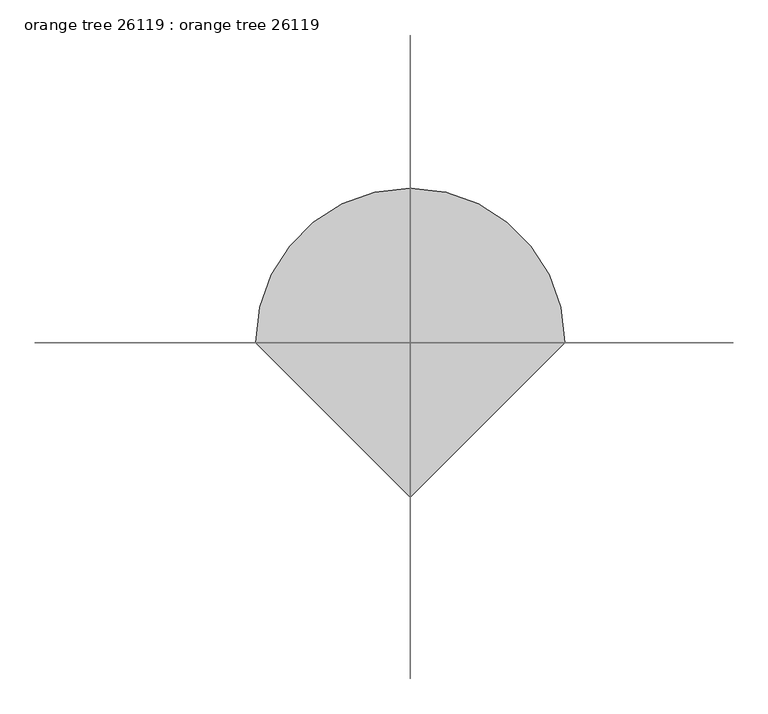
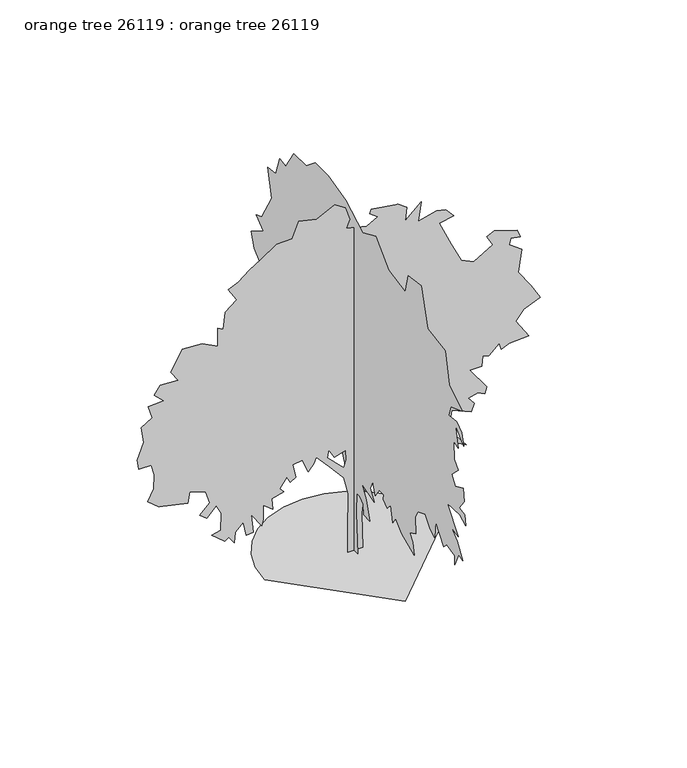
"""IFC4 building model written with IfcOpenShell, lengths in millimetres: proxy geometry, orange tree 26119 : orange tree 26119."""

import ifcopenshell
import ifcopenshell.guid

model = None  # the IFC model being written
_history = None  # IfcOwnerHistory: only IFC2X3 demands one
_inside = {}  # id of a spatial element -> (the spatial element, [elements in it])
_under = {}  # id of a project, library or spatial element -> (it, [spatial elements below it])
_declared = {}  # id of a project -> (the project, [libraries it declares])
_typed = {}  # id of a type object -> (the type object, [elements of that type])
_made_of = {}  # id of a material, layer set ... -> (it, [elements and type objects made of it])


def new_model(schema):
    """Start an empty IFC model of exactly this schema.

    Asked for "IFC4X3", IfcOpenShell would pick the latest addendum, in which some entities
    have other attributes; the version numbers below select the first issue.
    IFC2X3 requires an IfcOwnerHistory on every rooted entity: one is made here for all.
    """
    global model, _history
    if schema == "IFC4X3":
        model = ifcopenshell.file(schema_version=(4, 3, 0, 0))
    else:
        model = ifcopenshell.file(schema=schema)
    _inside.clear()
    _under.clear()
    _declared.clear()
    _typed.clear()
    _made_of.clear()
    _history = None
    if model.schema == "IFC2X3":
        org = make("IfcOrganization", Name="unknown")
        user = make(
            "IfcPersonAndOrganization",
            ThePerson=make("IfcPerson", FamilyName="unknown"),
            TheOrganization=org,
        )
        app = make(
            "IfcApplication",
            ApplicationDeveloper=org,
            Version="unknown",
            ApplicationFullName="unknown",
            ApplicationIdentifier="unknown",
        )
        _history = make(
            "IfcOwnerHistory",
            OwningUser=user,
            OwningApplication=app,
            ChangeAction="ADDED",
            CreationDate=0,
        )
    return model


def make(cls, **values):
    """One entity of the class cls with the attributes given. An attribute that is None is left unset."""
    return model.create_entity(
        cls, **{name: value for name, value in values.items() if value is not None}
    )


def rooted(cls, **values):
    """An entity with a GlobalId (a new one), such as an element, a storey or a relation."""
    return make(cls, GlobalId=ifcopenshell.guid.new(), OwnerHistory=_history, **values)


def si_unit(unit_type, name, prefix=None):
    """IfcSIUnit, for example si_unit("LENGTHUNIT", "METRE", prefix="MILLI")."""
    return make("IfcSIUnit", UnitType=unit_type, Prefix=prefix, Name=name)


def assignment(units):
    """IfcUnitAssignment: the units of a project."""
    return None if units is None else make("IfcUnitAssignment", Units=units)


def point(xyz):
    """IfcCartesianPoint."""
    return None if xyz is None else make("IfcCartesianPoint", Coordinates=xyz)


def direction(xyz):
    """IfcDirection."""
    return None if xyz is None else make("IfcDirection", DirectionRatios=xyz)


def frame(location, z_axis=None, x_axis=None):
    """IfcAxis2Placement3D, a coordinate frame: its origin and axes. An axis left out is left unset."""
    return make(
        "IfcAxis2Placement3D",
        Location=point(location),
        Axis=direction(z_axis),
        RefDirection=direction(x_axis),
    )


def origin():
    """The frame at (0, 0, 0) with its axes left unset."""
    return frame((0.0, 0.0, 0.0))


def place(relative_to, where):
    """IfcLocalPlacement: puts the frame where relative to a parent placement (None: the world)."""
    return make(
        "IfcLocalPlacement", PlacementRelTo=relative_to, RelativePlacement=where
    )


def context(
    kind, dimensions, precision=None, world=None, true_north=None, identifier=None
):
    """IfcGeometricRepresentationContext, for example the 3D "Model" context."""
    return make(
        "IfcGeometricRepresentationContext",
        ContextIdentifier=identifier,
        ContextType=kind,
        CoordinateSpaceDimension=dimensions,
        Precision=precision,
        WorldCoordinateSystem=world,
        TrueNorth=true_north,
    )


def project(units=None, contexts=None):
    """IfcProject with its units and contexts."""
    return rooted(
        "IfcProject",
        Name="project",
        RepresentationContexts=contexts,
        UnitsInContext=assignment(units),
    )


def spatial(cls, under=None, at=None, **own):
    """A site, building, storey or space (cls), placed at a placement, below another one or the project."""
    s = rooted(cls, ObjectPlacement=at, **own)
    if under is not None:
        _under.setdefault(under.id(), (under, []))[1].append(s)
    return s


def point_list(points):
    """IfcCartesianPointList2D or 3D."""
    cls = (
        "IfcCartesianPointList2D" if len(points[0]) == 2 else "IfcCartesianPointList3D"
    )
    return make(cls, CoordList=points)


def triangles(points, corners, closed=None, point_numbers=None):
    """IfcTriangulatedFaceSet: each triangle names its three corners, points numbered from 1."""
    return make(
        "IfcTriangulatedFaceSet",
        Coordinates=point_list(points),
        Closed=closed,
        CoordIndex=corners,
        PnIndex=point_numbers,
    )


def shape(context_of_items, identifier, shape_type, items):
    """IfcShapeRepresentation: the items that make up one representation, for example the "Body"."""
    return make(
        "IfcShapeRepresentation",
        ContextOfItems=context_of_items,
        RepresentationIdentifier=identifier,
        RepresentationType=shape_type,
        Items=items,
    )


def source(mapping_origin, context_of_items, identifier, shape_type, items):
    """IfcRepresentationMap: a shape defined once, which mapped items show again and again."""
    return make(
        "IfcRepresentationMap",
        MappingOrigin=mapping_origin,
        MappedRepresentation=shape(context_of_items, identifier, shape_type, items),
    )


def transform(
    local_origin,
    x_axis=None,
    y_axis=None,
    z_axis=None,
    scale=None,
    scale2=None,
    scale3=None,
    uniform=True,
):
    """IfcCartesianTransformationOperator3D, or its non-uniform kind. x_axis, y_axis, z_axis: its Axis1, 2, 3."""
    if uniform:
        return make(
            "IfcCartesianTransformationOperator3D",
            Axis1=direction(x_axis),
            Axis2=direction(y_axis),
            LocalOrigin=point(local_origin),
            Scale=scale,
            Axis3=direction(z_axis),
        )
    return make(
        "IfcCartesianTransformationOperator3DnonUniform",
        Axis1=direction(x_axis),
        Axis2=direction(y_axis),
        LocalOrigin=point(local_origin),
        Scale=scale,
        Axis3=direction(z_axis),
        Scale2=scale2,
        Scale3=scale3,
    )


def mapped(mapping_source, mapping_target):
    """IfcMappedItem: shows the shape of a source again, moved by a transform."""
    return make(
        "IfcMappedItem", MappingSource=mapping_source, MappingTarget=mapping_target
    )


def made_of(thing, what):
    """Note that an element or type object is made of a material, layer set ...; save() writes the relation."""
    if what is not None:
        _made_of.setdefault(what.id(), (what, []))[1].append(thing)
    return thing


def element(
    cls,
    number,
    at=None,
    inside=None,
    cuts=None,
    type_object=None,
    material=None,
    context=None,
    identifier="Body",
    shape_type=None,
    held_by="IfcProductDefinitionShape",
    body=None,
    shapes=None,
    **own,
):
    """One element of the class cls, such as IfcWall. Its Tag is "e" and its number.

    at: its placement. inside: the storey or other place that contains it. cuts: it is an
    opening in that element (IfcRelVoidsElement). A single representation is given by context,
    identifier, shape_type and body (its items); several are given by shapes. held_by: the class
    of the entity that holds the representations. save() writes the other relations.
    """
    e = rooted(cls, Tag="e%d" % number, ObjectPlacement=at, **own)
    if body is not None:
        shapes = [shape(context, identifier, shape_type, body)]
    if shapes is not None:
        e.Representation = make(held_by, Representations=shapes)
    if inside is not None:
        _inside.setdefault(inside.id(), (inside, []))[1].append(e)
    if cuts is not None:
        rooted(
            "IfcRelVoidsElement", RelatingBuildingElement=cuts, RelatedOpeningElement=e
        )
    if type_object is not None:
        _typed.setdefault(type_object.id(), (type_object, []))[1].append(e)
    return made_of(e, material)


def aggregate(whole, parts):
    """IfcRelAggregates: a whole, such as a stair, and the parts it consists of."""
    return rooted("IfcRelAggregates", RelatingObject=whole, RelatedObjects=parts)


def save(model, path):
    """Write the relations noted so far, then the file.

    IfcRelAggregates (storeys below a building ...), IfcRelContainedInSpatialStructure (elements
    in a storey), IfcRelDefinesByType, IfcRelAssociatesMaterial and IfcRelDeclares: one each for
    every whole, place, type object, material and project.
    """
    for whole, parts in _under.values():
        aggregate(whole, parts)
    for where, things in _inside.values():
        rooted(
            "IfcRelContainedInSpatialStructure",
            RelatedElements=things,
            RelatingStructure=where,
        )
    for kind, things in _typed.values():
        rooted("IfcRelDefinesByType", RelatedObjects=things, RelatingType=kind)
    for what, things in _made_of.values():
        rooted("IfcRelAssociatesMaterial", RelatedObjects=things, RelatingMaterial=what)
    for by, libraries in _declared.values():
        rooted("IfcRelDeclares", RelatingContext=by, RelatedDefinitions=libraries)
    model.write(path)


def orange_tree_26119_orange_tree_26119_f1cce5cf(model_context):
    return source(origin(), model_context, "Body", "Tessellation", [
        triangles([(-803.9534712, 0.0, 6.05e-05), (-782.6987366, 184.2127929, 6.05e-05), (-722.1679836, 353.3826814, 6.05e-05), (-627.2075008, 502.663613, 6.05e-05), (-502.663613, 627.2075008, 6.05e-05), (-353.3826814, 722.1679836, 6.05e-05), (-184.2125386, 782.6987366, 6.05e-05), (3.51e-05, 803.9534712, 6.05e-05), (184.2127929, 782.6987366, 6.05e-05), (353.3826814, 722.1679836, 6.05e-05), (502.663613, 627.2075008, 6.05e-05), (627.2075008, 502.663613, 6.05e-05), (722.1679836, 353.3826814, 6.05e-05), (782.6987366, 184.2125386, 6.05e-05), (803.9534712, -7.03e-05, 6.05e-05), (-0.0001054, -803.9534712, 6.05e-05), (-4.73e-05, 77.0963933, 4.81e-05), (-2.95e-05, 72.7562921, 588.9525321), (-2.7e-05, 181.2628458, 836.3460434), (-3.2e-05, 320.1518609, 875.4087753), (-3.63e-05, 346.1919502, 771.2433311), (-3.87e-05, 472.0617019, 879.7495714), (-4.71e-05, 532.8235817, 688.7770712), (-4.92e-05, 632.6507006, 766.9024624), (-5.78e-05, 693.4151602, 571.5916368), (-5.81e-05, 775.878804, 684.4387459), (-6.3e-05, 832.3023949, 606.3134274), (-6.59e-05, 979.8713671, 727.8398031), (-5.62e-05, 875.7059229, 897.110503), (-4.32e-05, 610.9489002, 936.1731623), (-5.12e-05, 849.6633265, 1027.3185436), (-5.75e-05, 1031.9540892, 1088.0830032), (-6.35e-05, 1166.5029985, 1088.0830032), (-6.17e-05, 1201.224789, 1200.9301849), (-6.47e-05, 1296.7111118, 1244.3311695), (-5.59e-05, 1244.6283897, 1461.3462662), (-6.14e-05, 1422.5782837, 1543.8099827), (-6.28e-05, 1578.8289207, 1730.4416142), (-5.38e-05, 1452.9591328, 1843.2887959), (-5.55e-05, 1552.7863243, 1938.7749733), (-5.37e-05, 1600.5281776, 2068.9830139), (-4.21e-05, 1418.2374149, 2186.1685936), (-4.43e-05, 1526.7437279, 2272.9730335), (-3.95e-05, 1439.9391426, 2303.3564987), (-2.42e-05, 1279.3501076, 2576.8055054), (-1.94e-05, 1344.4529652, 2837.2061806), (-1.34e-05, 1218.5857206, 2850.2364899), (-5.3e-06, 1157.821261, 3028.1889999), (-1.5e-06, 1062.3375544, 3015.1586906), (9.7e-06, 940.8087078, 3206.14151), (1.89e-05, 741.1570135, 3214.8028999), (2.81e-05, 606.6080678, 3323.3116837), (3.75e-05, 398.2746723, 3327.6550232), (4.77e-05, 124.839264, 3258.2115875), (5.48e-05, -135.5766083, 3106.2941162), (6.66e-05, -339.5701524, 3197.4545403), (6.98e-05, -543.560172, 2997.8106216), (7.98e-05, -799.6379642, 2950.0585945), (8.73e-05, -847.3798176, 3128.0111046), (9.73e-05, -1051.3723806, 3158.3894829), (9.14e-05, -1151.1994995, 2811.1714325), (0.0001025, -1428.9739689, 2767.7627449), (9.64e-05, -1485.3975597, 2476.9656693), (0.0001018, -1689.3900501, 2351.0983521), (9.21e-05, -1515.7810249, 2285.9956398), (8.75e-05, -1481.0591618, 2186.1685936), (9.36e-05, -1606.926479, 2199.1910545), (9.54e-05, -1685.0517975, 2142.767609), (9.34e-05, -1715.4327919, 2029.9204273), (9.11e-05, -1580.8837372, 2155.7875992), (8.77e-05, -1632.9664593, 1964.815099), (8.51e-05, -1559.1820095, 1986.5168266), (8.02e-05, -1563.5228783, 1817.2460541), (8.14e-05, -1632.9664593, 1752.1433418), (7.34e-05, -1524.4602917, 1647.9754269), (7.38e-05, -1585.2246059, 1569.8525791), (8.13e-05, -1711.0919231, 1630.6144226), (7.79e-05, -1719.7736607, 1504.7472507), (7.16e-05, -1645.9890656, 1404.9226753), (7.48e-05, -1728.4527821, 1387.5618164), (7.27e-05, -1745.813641, 1292.0754936), (6.99e-05, -1650.3299343, 1339.817347), (6.11e-05, -1459.3574341, 1331.1382256), (6.23e-05, -1628.6282066, 1118.463925), (5.81e-05, -1520.1218937, 1140.1657253), (5.99e-05, -1611.2673477, 1062.0404068), (5.99e-05, -1698.0717876, 931.8322935), (5.77e-05, -1637.307328, 949.1932251), (5.11e-05, -1576.5454845, 818.9851845), (5.33e-05, -1572.2046158, 901.4513718), (4.88e-05, -1450.6756966, 931.8322935), (4.52e-05, -1402.9338432, 884.0904402), (4.47e-05, -1281.4075401, 1049.020344), (3.92e-05, -1264.0440651, 888.4313089), (3.71e-05, -1194.6004841, 923.1530994), (3.64e-05, -1116.4751656, 1018.6394222), (2.99e-05, -999.2896585, 975.2358215), (2.55e-05, -955.8861305, 892.7696342), (2.14e-05, -964.567868, 740.8623367), (1.6e-05, -873.4224867, 697.4588087), (1.6e-05, -916.8234713, 632.353553), (1.37e-05, -938.5251989, 523.8472401), (7.6e-06, -743.2143734, 610.6542961), (6.3e-06, -656.4073174, 697.4588087), (2.2e-06, -608.665464, 632.353553), (5.3e-06, -578.2845423, 779.9225252), (9e-07, -521.8609514, 719.1606091), (-7e-07, -456.7556594, 762.5615936), (1.1e-06, -465.4373606, 810.3059904), (-2e-06, -395.9937432, 810.3059904), (-7.3e-06, -335.22932, 723.5014778), (-6e-06, -291.8257738, 832.0077181), (-1e-05, -257.1039651, 749.5415308), (-1.02e-05, -317.8683884, 649.7169554), (-1.72e-05, -122.5560549, 710.4788715), (-1.74e-05, -192.000181, 597.6317262), (-2.03e-05, -244.0831574, 424.0226646), (-2.39e-05, -157.2781179, 432.7018224), (-2.16e-05, -144.2573102, 528.1880725), (-2.27e-05, -92.1740885, 571.5916368), (-2.48e-05, -44.4312178, 571.5916368), (-3.04e-05, -40.0908669, 389.3008378), (-4.11e-05, -61.7923765, 5.22e-05), (-2.23e-05, 137.8603261, 927.4914248), (-2.41e-05, 124.8395184, 849.3686497), (-2.39e-05, 33.6941257, 719.1606091), (-1.71e-05, 3.3121102, 901.4513718), (-1.8e-05, 64.07584, 962.2158314), (58.7260893, -2.69e-05, 920.6994701), (38.9260215, -3.03e-05, 877.8014345), (32.3258294, -4.22e-05, 683.1001648), (45.5259593, -4.5e-05, 626.9992287), (78.5256484, -3.59e-05, 755.7010386), (104.9259083, -2.72e-05, 881.1008698), (-56.7740963, -8.68e-05, 0.0), (-53.4738754, -7.45e-05, 204.6001204), (-50.1739042, -5.35e-05, 554.4008984), (-93.0740155, -4.51e-05, 726.0008165), (-225.0743068, -4.16e-05, 881.1008698), (-337.2739989, -3.93e-05, 1003.2012657), (-363.6747857, -4.36e-05, 950.3996922), (-409.8748363, -4.89e-05, 894.3012995), (-465.9733017, -4.39e-05, 1019.7011307), (-551.7745325, -4.85e-05, 1006.500701), (-522.0743105, -5.46e-05, 881.1008698), (-574.8733043, -5.89e-05, 848.1012125), (-604.5735263, -5.67e-05, 907.4991131), (-667.2734419, -6.47e-05, 818.4009905), (-634.2737846, -6.56e-05, 778.799774), (-739.8743156, -7.2e-05, 749.099552), (-729.9733938, -7.77e-05, 646.8010723), (-819.0740599, -7.74e-05, 716.0998947), (-815.7746246, -8.54e-05, 580.7991417), (-832.2744169, -8.94e-05, 524.7006763), (-924.6745909, -8.52e-05, 663.3008646), (-904.8752907, -9.48e-05, 488.3989677), (-970.8746778, -9.8e-05, 481.8000609), (-997.2754646, -9.11e-05, 617.1008503), (-1069.8737223, -9.86e-05, 544.4999765), (-1079.7746441, -0.0001046, 452.0998389), (-1129.2741663, -0.0001028, 518.0991898), (-1165.5758749, -0.0001058, 495.0004543), (-1281.0748569, -0.0001051, 590.7000635), (-1201.8750401, -0.0001005, 610.4993637), (-1195.2735535, -9.05e-05, 772.2009035), (-1241.4736404, -8.73e-05, 861.2990261), (-1327.2749439, -9.65e-05, 768.9013956), (-1389.9747505, -9.61e-05, 821.7004257), (-1300.8740845, -8.71e-05, 907.4991131), (-1337.1733223, -8.2e-05, 1019.7011307), (-1479.0755619, -8.49e-05, 1075.799596), (-1495.5752815, -9.19e-05, 970.2015358), (-1759.5754463, -9.97e-05, 1032.9014877), (-1858.5744907, -9.91e-05, 1115.4007399), (-1805.7755333, -9.07e-05, 1217.6992195), (-1799.1740467, -8.25e-05, 1349.70061), (-1825.5747608, -7.76e-05, 1451.999017), (-1937.7743076, -8.27e-05, 1448.6996544), (-1950.9746647, -7.78e-05, 1541.0998283), (-1894.8735832, -6.63e-05, 1692.9004463), (-1917.9749348, -5.84e-05, 1841.4015564), (-1815.6739117, -5.04e-05, 1900.7993843), (-1855.2749828, -4.52e-05, 2016.3009098), (-1713.3753593, -3.86e-05, 2022.8997803), (-1799.1740467, -3.75e-05, 2105.4015759), (-1746.3750893, -3.05e-05, 2184.6013927), (-1584.6734768, -2.4e-05, 2174.7003983), (-1650.6754074, -2.1e-05, 2273.6994427), (-1548.3743843, -5.5e-06, 2458.4999359), (-1366.8735443, 1.9e-06, 2448.6014122), (-1228.2732834, 3.6e-06, 2376.0006111), (-1228.2732834, 1.38e-05, 2547.5953697), (-1178.7737612, 1.44e-05, 2521.1995972), (-1158.974461, 2.45e-05, 2676.2973976), (-1056.6733652, 3.39e-05, 2758.7964317), (-1132.5736742, 3.79e-05, 2880.8942116), (-1040.1735003, 4.41e-05, 2917.1908333), (-941.1744558, 5.33e-05, 2999.6901581), (-835.5739248, 6.19e-05, 3065.7047333), (-693.6742287, 7.36e-05, 3158.1101395), (-555.0740041, 7.98e-05, 3161.4119728), (-495.6735237, 9.13e-05, 3309.9005836), (-333.9745637, 9.62e-05, 3273.6039619), (-172.2735144, 0.000108, 3352.8011627), (-79.8736311, 0.0001083, 3290.0884209), (-36.9737765, 0.0001029, 3167.990641), (-66.673751, 9.71e-05, 3092.0952736), (114.8263214, 0.0001024, 3049.1946945), (213.8264105, 0.0001101, 3105.303479), (144.5262982, 0.00011, 3154.8080154), (154.426457, 0.0001128, 3194.4067612), (401.9271747, 0.0001213, 3154.8080154), (477.8274837, 0.0001215, 3102.001355), (461.327655, 0.0001133, 2976.6014511), (606.5267864, 0.0001275, 3108.6053123), (580.126036, 0.0001159, 2933.700872), (745.1270473, 0.0001255, 2973.2996178), (827.6262268, 0.0001279, 2953.5130348), (900.2271006, 0.0001263, 2874.2902542), (768.2257828, 0.000119, 2847.8997139), (877.125749, 0.0001096, 2610.3081116), (929.9273226, 0.0001052, 2498.1010071), (969.525923, 0.0001024, 2422.2006981), (1078.4258892, 0.0001042, 2372.7011032), (1253.3278587, 0.000118, 2474.9995102), (1197.2268499, 0.0001212, 2570.7093658), (1266.525745, 0.000126, 2600.4020302), (1474.4272991, 0.0001312, 2534.4002449), (1497.5260345, 0.0001279, 2461.8017693), (1415.0268551, 0.0001252, 2478.3016342), (1401.826498, 0.0001211, 2418.9011902), (1514.0258995, 0.0001213, 2339.7013733), (1481.0261696, 0.0001075, 2131.7998192), (1593.2257164, 0.0001027, 1970.1008228), (1679.0268745, 9.78e-05, 1824.9016914), (1530.5257645, 8.76e-05, 1762.1992687), (1457.9274342, 7.91e-05, 1673.1010735), (1576.7258514, 7.35e-05, 1491.6002335), (1398.5269901, 6.51e-05, 1481.6993843), (1329.2255516, 6.03e-05, 1451.999017), (1309.4263241, 6.32e-05, 1514.701585), (1213.7267149, 5.39e-05, 1428.9002815), (1160.9276848, 5.24e-05, 1442.1006386), (1151.026763, 4.66e-05, 1352.9999725), (1045.426232, 4.18e-05, 1349.70061), (1197.2268499, 3.59e-05, 1138.4994753), (1180.726985, 3.16e-05, 1079.1015747), (1114.7275978, 3.05e-05, 1108.7992533), (1032.2258749, 2.57e-05, 1088.9999531), (1085.0273758, 2.39e-05, 1019.7011307), (1058.626589, 1.86e-05, 950.3996922), (883.7272356, 1.53e-05, 1023.0005659), (854.0270136, 3.8e-06, 851.4006477), (1012.4265747, -1.3e-06, 650.1005075), (877.125749, -2.7e-06, 726.0008165), (830.9257347, -1.63e-05, 531.2995831), (801.2255127, -1.04e-05, 653.3999428), (745.1270473, -8.7e-06, 722.7013813), (642.8259516, -1.59e-05, 676.5012943), (586.7274862, -2.47e-05, 570.900727), (487.725862, -2.15e-05, 696.3005945), (392.0262528, -1.76e-05, 831.6013475), (349.1256374, -2.48e-05, 742.5006815), (316.1259439, -1.76e-05, 887.6998129), (187.4264049, -2.7e-05, 824.999861), (114.8263214, -3.72e-05, 706.1989729), (71.9262193, -6.15e-05, 329.999443), (81.8261282, -8.08e-05, 0.0001067), (-178.8742198, -3.57e-05, 947.1002569), (-228.3742689, -3.25e-05, 1036.200923), (-238.2741733, -3.73e-05, 963.6001219), (-89.7740443, -3.95e-05, 818.4009905), (-66.6740053, -3.43e-05, 887.6998129), (-73.2739431, -2.91e-05, 980.0999868)], [[16, 15, 1], [15, 14, 1], [1, 14, 2], [14, 13, 2], [2, 13, 3], [3, 13, 4], [13, 12, 4], [12, 11, 4], [4, 11, 5], [5, 11, 6], [6, 11, 7], [7, 11, 8], [8, 11, 9], [9, 11, 10], [17, 126, 18], [89, 88, 90], [69, 68, 70], [68, 67, 70], [84, 83, 85], [87, 86, 88], [18, 126, 19], [126, 125, 19], [114, 113, 115], [105, 104, 106], [64, 63, 65], [81, 80, 82], [80, 79, 82], [67, 66, 70], [25, 24, 26], [102, 101, 103], [111, 110, 112], [43, 42, 44], [71, 70, 72], [21, 20, 22], [101, 100, 103], [117, 116, 118], [118, 116, 119], [77, 76, 78], [23, 22, 24], [94, 93, 95], [95, 93, 96], [78, 76, 79], [92, 91, 93], [46, 45, 47], [119, 116, 120], [116, 115, 120], [27, 26, 28], [28, 26, 29], [29, 26, 30], [26, 24, 30], [24, 22, 30], [17, 123, 126], [123, 122, 126], [122, 121, 126], [74, 73, 75], [82, 79, 83], [79, 76, 83], [38, 37, 39], [125, 124, 19], [60, 59, 61], [59, 58, 61], [107, 106, 108], [108, 106, 109], [70, 66, 72], [19, 124, 20], [35, 34, 36], [48, 47, 49], [103, 100, 104], [120, 115, 121], [121, 115, 126], [126, 115, 127], [41, 40, 42], [40, 39, 42], [33, 32, 34], [115, 113, 127], [113, 112, 127], [62, 61, 63], [56, 55, 57], [99, 98, 100], [100, 98, 104], [104, 98, 106], [88, 86, 90], [90, 86, 91], [86, 85, 91], [91, 85, 93], [85, 83, 93], [76, 75, 83], [37, 36, 39], [50, 49, 51], [93, 83, 96], [34, 32, 36], [98, 97, 106], [32, 31, 36], [44, 42, 45], [106, 97, 109], [52, 51, 53], [83, 75, 96], [96, 75, 97], [63, 61, 65], [65, 61, 66], [61, 58, 66], [58, 57, 66], [97, 75, 109], [75, 73, 109], [73, 72, 109], [72, 66, 109], [66, 57, 109], [109, 57, 110], [110, 57, 112], [112, 57, 127], [127, 57, 128], [57, 55, 128], [55, 54, 128], [54, 53, 128], [53, 51, 128], [51, 49, 128], [49, 47, 128], [47, 45, 128], [45, 42, 128], [42, 39, 128], [39, 36, 128], [36, 31, 128], [31, 30, 128], [128, 30, 124], [124, 30, 20], [20, 30, 22], [130, 135, 131], [135, 130, 136], [136, 130, 137], [131, 135, 132], [254, 253, 255], [256, 255, 257], [137, 130, 138], [129, 272, 130], [130, 272, 138], [272, 129, 273], [263, 262, 264], [215, 214, 216], [138, 272, 139], [272, 271, 139], [139, 271, 140], [160, 159, 161], [151, 150, 152], [154, 153, 155], [153, 152, 155], [163, 162, 164], [219, 218, 220], [238, 237, 239], [229, 228, 230], [228, 227, 230], [192, 191, 193], [142, 141, 143], [149, 148, 150], [260, 259, 261], [183, 182, 184], [218, 217, 220], [162, 161, 164], [271, 270, 140], [273, 129, 274], [196, 195, 197], [135, 268, 132], [268, 267, 132], [267, 266, 132], [132, 266, 133], [266, 265, 133], [133, 265, 134], [247, 246, 248], [246, 245, 248], [235, 234, 236], [141, 140, 143], [226, 225, 227], [227, 225, 230], [230, 225, 231], [168, 167, 169], [167, 166, 169], [240, 239, 241], [146, 145, 147], [145, 144, 147], [257, 255, 258], [255, 253, 258], [172, 171, 173], [239, 237, 241], [217, 216, 220], [248, 245, 249], [251, 250, 252], [250, 249, 252], [156, 155, 157], [157, 155, 158], [211, 210, 212], [210, 209, 212], [178, 177, 179], [244, 243, 245], [202, 201, 203], [185, 184, 186], [186, 184, 187], [269, 274, 270], [174, 173, 175], [173, 171, 175], [161, 159, 164], [179, 177, 180], [159, 158, 164], [164, 158, 165], [158, 155, 165], [175, 171, 176], [181, 180, 182], [189, 188, 190], [188, 187, 190], [190, 187, 191], [232, 231, 233], [249, 245, 252], [213, 212, 214], [212, 209, 214], [204, 203, 205], [205, 203, 206], [206, 203, 207], [203, 201, 207], [265, 264, 134], [209, 208, 214], [242, 241, 243], [231, 225, 233], [225, 224, 233], [234, 233, 236], [233, 224, 236], [236, 224, 237], [237, 224, 241], [241, 224, 243], [224, 223, 243], [243, 223, 245], [155, 152, 165], [165, 152, 166], [261, 259, 262], [259, 258, 262], [258, 253, 262], [253, 252, 262], [262, 252, 264], [252, 245, 264], [245, 223, 264], [264, 223, 134], [134, 223, 129], [129, 223, 274], [274, 223, 270], [223, 222, 270], [222, 221, 270], [221, 220, 270], [220, 216, 270], [216, 214, 270], [214, 208, 270], [208, 207, 270], [207, 201, 270], [201, 200, 270], [200, 199, 270], [199, 198, 270], [198, 197, 270], [197, 195, 270], [195, 194, 270], [194, 193, 270], [193, 191, 270], [270, 191, 140], [140, 191, 143], [143, 191, 144], [191, 187, 144], [187, 184, 144], [184, 182, 144], [182, 180, 144], [180, 177, 144], [177, 176, 144], [176, 171, 144], [171, 170, 144], [144, 170, 147], [170, 169, 147], [169, 166, 147], [166, 152, 147], [147, 152, 148], [148, 152, 150]], closed=False),
    ])


if __name__ == "__main__":
    model = new_model("IFC4")
    model_context = context("Model", 3, world=origin())
    ifc_project = project(units=[si_unit("LENGTHUNIT", "METRE", prefix="MILLI")], contexts=[model_context])
    site = spatial("IfcSite", under=ifc_project)
    building = spatial("IfcBuilding", under=site)
    placement = place(None, origin())
    orange_tree_26119_orange_tree_26119_shape = orange_tree_26119_orange_tree_26119_f1cce5cf(model_context)
    element("IfcBuildingElementProxy", 1, Name="orange tree 26119 : orange tree 26119", ObjectType="orange tree 26119 : orange tree 26119", at=placement, inside=building, context=model_context, shape_type="MappedRepresentation", body=[
        mapped(orange_tree_26119_orange_tree_26119_shape, transform((0.0, 0.0, 0.0), x_axis=(1.0, 0.0, 0.0), y_axis=(0.0, 1.0, 0.0), z_axis=(0.0, 0.0, 1.0))),
    ])
    save(model, "model.ifc")

# Revit data of these elements
# Type "orange tree 26119 : orange tree 26119"
#   built-in parameter 1005195 = "RPC-16-FVGW-4XXX-7J75-W000-ST1L-LVER-AU"
#   Height = 0
